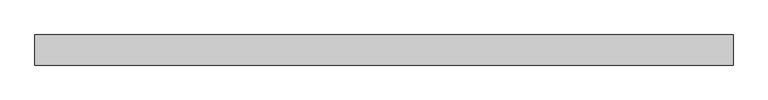
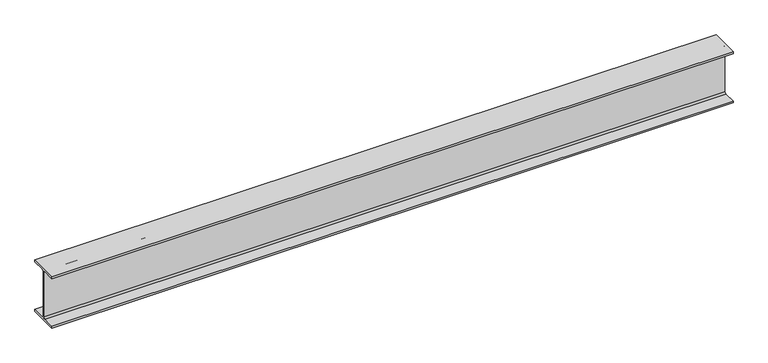
"""IFC4 building model written with IfcOpenShell, lengths in millimetres: beam geometry, Old_Steel Beam_H-KSD3502 : H_SB_ASB_H-200×200x8x12."""

from ifc_helpers import new_model, si_unit, point, frame, frame_2d, origin, place, context, project, spatial, polyline, circle_curve, trimmed, segment, composite_curve, outline, extrude, source, transform, mapped, element, save


def beam_15115ed1(model_context):
    return source(origin(), model_context, "Body", "SweptSolid", [
        extrude(outline(composite_curve([segment(polyline([(82.5, -141.5), (82.5, -151.7), (-82.5, -151.7), (-82.5, -141.5), (-11.9, -141.5)]), True, "CONTINUOUS"), segment(trimmed(circle_curve(frame_2d((-11.9, -132.6)), 8.9), [point((-11.9, -141.5))], [point((-3.0, -132.6))], True, "CARTESIAN"), True, "CONTINUOUS"), segment(polyline([(-3.0, -132.6), (-3.0, 132.6)]), True, "CONTINUOUS"), segment(trimmed(circle_curve(frame_2d((-11.9, 132.6)), 8.9), [point((-3.0, 132.6))], [point((-11.9, 141.5))], True, "CARTESIAN"), True, "CONTINUOUS"), segment(polyline([(-11.9, 141.5), (-82.5, 141.5), (-82.5, 151.7), (82.5, 151.7), (82.5, 141.5), (11.9, 141.5)]), True, "CONTINUOUS"), segment(trimmed(circle_curve(frame_2d((11.9, 132.6)), 8.9), [point((11.9, 141.5))], [point((3.0, 132.6))], True, "CARTESIAN"), True, "CONTINUOUS"), segment(polyline([(3.0, 132.6), (3.0, -132.6)]), True, "CONTINUOUS"), segment(trimmed(circle_curve(frame_2d((11.9, -132.6)), 8.9), [point((3.0, -132.6))], [point((11.9, -141.5))], True, "CARTESIAN"), True, "CONTINUOUS"), segment(polyline([(11.9, -141.5), (82.5, -141.5)]), True, "CONTINUOUS")], self_intersect=False)), frame((-1998.6606017, 0.0, 0.0), z_axis=(1.0, 0.0, 0.0), x_axis=(0.0, 1.0, 0.0)), (0.0, 0.0, 1.0), 3820.5090386),
    ])


if __name__ == "__main__":
    model = new_model("IFC4")
    model_context = context("Model", 3, world=origin())
    ifc_project = project(units=[si_unit("LENGTHUNIT", "METRE", prefix="MILLI")], contexts=[model_context])
    site = spatial("IfcSite", under=ifc_project)
    building = spatial("IfcBuilding", under=site)
    placement = place(None, origin())
    beam_shape = beam_15115ed1(model_context)
    element("IfcBeam", 1, ObjectType="Old_Steel Beam_H-KSD3502 : H_SB_ASB_H-200×200x8x12", at=placement, inside=building, context=model_context, shape_type="MappedRepresentation", body=[
        mapped(beam_shape, transform((0.0, 0.0, 0.0), x_axis=(1.0, 0.0, 0.0), y_axis=(0.0, 1.0, 0.0), z_axis=(0.0, 0.0, 1.0))),
    ])
    save(model, "model.ifc")

# Revit data of these elements
# Type "Old_Steel Beam_H-KSD3502 : H_SB_ASB_H-200×200x8x12"
#   Width = 20.0 cm
#   Web Thickness = 0.8 cm
#   Web Fillet = 1.3 cm
#   Warping Constant = 141376.0 cm⁶
#   Torsional Moment of Inertia = 26.2485 cm⁴
#   Torsional Modulus = 1.0 cm³
#   Section Area = 63.53 cm²
#   Plastic Modulus weak axis = 244.0 cm³
#   Plastic Modulus strong axis = 525.0 cm³
#   Perimeter = 1.16 m²/m
#   Nominal Weight = 49.90 kgf/m
#   Moment of Inertia weak axis = 1600.00 cm⁴
#   Moment of Inertia strong axis = 4720.00 cm⁴
#   Height = 20.0 cm
#   Flange Thickness = 1.2 cm
#   Elastic Modulus weak axis = 160.0 cm³
#   Elastic Modulus strong axis = 472.0 cm³
#   Centroid Vertical = 10.0 cm
#   Centroid Horizontal = 10.0 cm
#   Length [instance default] = 1.5240 m
#   Structural Material [instance default] = Steel, 45-345
#   Assembly Code = ""
# Element 1 (IfcBeam, "Old_Steel Beam_H-KSD3502 : H_SB_ASB_H-200×200x8x12")
#   Structural Material = none
# Materials
#   "Steel, 45-345": class "Metal", colour RGB 189 187 185, transparency 0, Description = "Steel 345 MPa", Cost = 0
